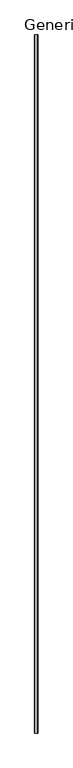
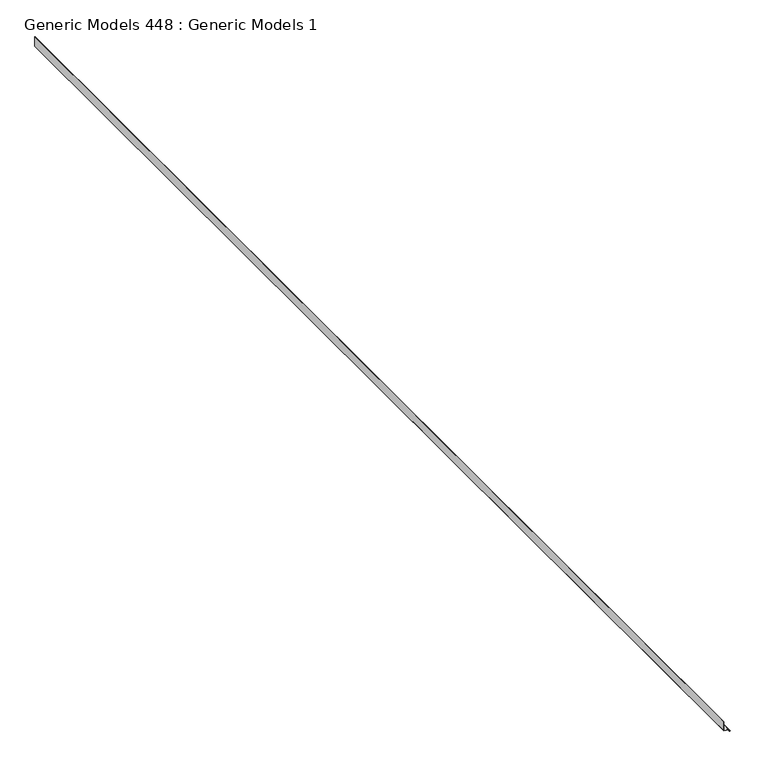
"""IFC4 building model written with IfcOpenShell, lengths in millimetres: proxy geometry, Generic Models 448 : Generic Models 1."""

from ifc_helpers import new_model, si_unit, point, frame, frame_2d, origin, place, context, project, spatial, polyline, circle_curve, trimmed, segment, composite_curve, outline, extrude, source, transform, mapped, element, save


def generic_models_448_generic_models_1_a9e192d1(model_context):
    return source(origin(), model_context, "Body", "SweptSolid", [
        extrude(outline(composite_curve([segment(polyline([(126242.2799075, 1714.4975778), (126239.5333743, 1745.8905959), (126231.6756502, 1753.74832)]), True, "CONTINUOUS"), segment(trimmed(circle_curve(frame_2d((126230.5531182, 1752.625788)), 1.5875), [point((126231.6756502, 1753.74832))], [point((126229.4305862, 1753.74832))], True, "CARTESIAN"), True, "CONTINUOUS"), segment(polyline([(126229.4305862, 1753.74832), (126228.8693201, 1753.187054)]), True, "CONTINUOUS"), segment(trimmed(circle_curve(frame_2d((126229.9918522, 1752.0645219)), 1.5875), [point((126228.8693201, 1753.187054))], [point((126228.8693201, 1750.9419899))], True, "CARTESIAN"), True, "CONTINUOUS"), segment(polyline([(126228.8693201, 1750.9419899), (126236.7270443, 1743.0842658), (126236.1657782, 1742.5229998), (126228.3080541, 1750.3807239)]), True, "CONTINUOUS"), segment(trimmed(circle_curve(frame_2d((126229.9918522, 1752.0645219)), 2.38125), [point((126228.3080541, 1750.3807239))], [point((126228.3080541, 1753.74832))], False, "CARTESIAN"), True, "CONTINUOUS"), segment(polyline([(126228.3080541, 1753.74832), (126228.8693201, 1754.309586)]), True, "CONTINUOUS"), segment(trimmed(circle_curve(frame_2d((126230.5531182, 1752.625788)), 2.38125), [point((126228.8693201, 1754.309586))], [point((126232.2369162, 1754.309586))], False, "CARTESIAN"), True, "CONTINUOUS"), segment(polyline([(126232.2369162, 1754.309586), (126240.2989244, 1746.2475778), (126243.0072454, 1715.2913278), (126305.7799075, 1715.2913278), (126305.7799075, 1714.4975778), (126242.2799075, 1714.4975778)]), True, "CONTINUOUS")], self_intersect=False)), frame((0.0, 306.6963299, 0.0), z_axis=(0.0, 1.0, 0.0), x_axis=(0.0, 0.0, 1.0)), (0.0, 0.0, 1.0), 7886.7),
    ])


if __name__ == "__main__":
    model = new_model("IFC4")
    model_context = context("Model", 3, world=origin())
    ifc_project = project(units=[si_unit("LENGTHUNIT", "METRE", prefix="MILLI")], contexts=[model_context])
    site = spatial("IfcSite", under=ifc_project)
    building = spatial("IfcBuilding", under=site)
    placement = place(None, origin())
    generic_models_448_generic_models_1_shape = generic_models_448_generic_models_1_a9e192d1(model_context)
    element("IfcBuildingElementProxy", 1, Name="Generic Models 448 : Generic Models 1", ObjectType="Generic Models 448 : Generic Models 1", at=placement, inside=building, context=model_context, shape_type="MappedRepresentation", body=[
        mapped(generic_models_448_generic_models_1_shape, transform((0.0, 0.0, 0.0), x_axis=(1.0, 0.0, 0.0), y_axis=(0.0, 1.0, 0.0), z_axis=(0.0, 0.0, 1.0))),
    ])
    save(model, "model.ifc")

# Revit data of these elements
# Element 1 (IfcBuildingElementProxy, "Generic Models 448 : Generic Models 1")
#   Materials on its faces: "_CONT. 16 GA. COPPER DRIP FLASHING"
# Materials
#   "_CONT. 16 GA. COPPER DRIP FLASHING": class "Metal", colour RGB 199 199 199, transparency 0, Description = "Structural steel 50ksi", Cost = 0
